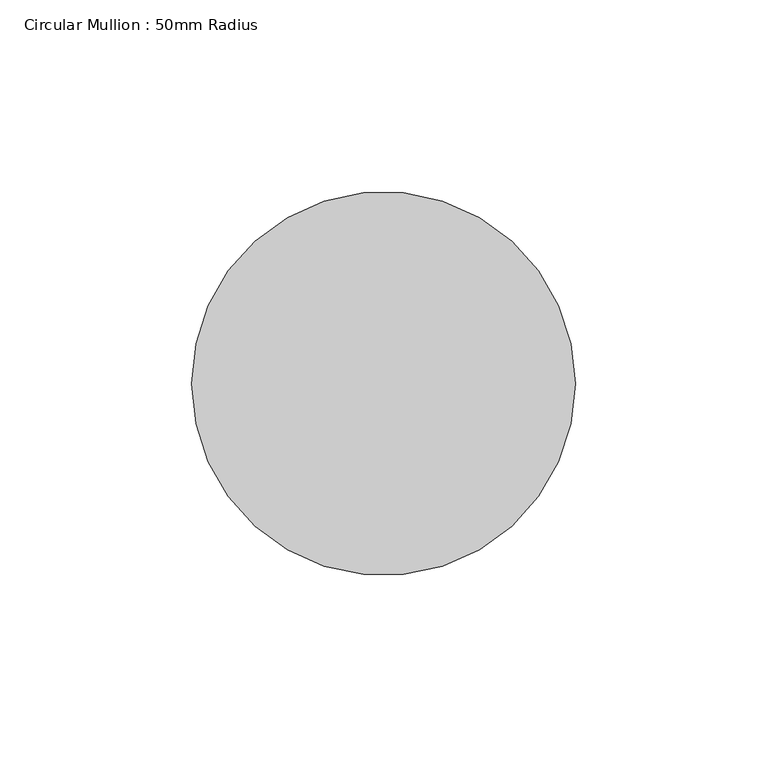
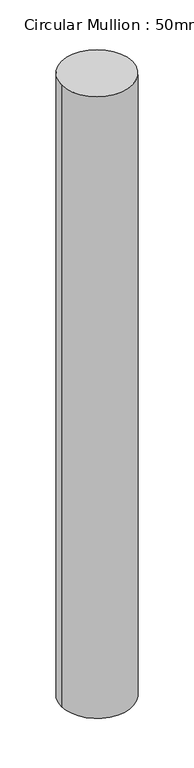
"""IFC4 building model written with IfcOpenShell, lengths in millimetres: member geometry, Circular Mullion : 50mm Radius."""

from ifc_helpers import new_model, si_unit, point, frame, origin, origin_2d, place, context, project, spatial, circle_curve, trimmed, segment, composite_curve, outline, extrude, source, transform, mapped, element, save


def circular_mullion_50mm_radius_4ba9e032(model_context):
    return source(origin(), model_context, "Body", "SweptSolid", [
        extrude(outline(composite_curve([segment(trimmed(circle_curve(origin_2d(), 50.0), [point((50.0, 0.0))], [point((-50.0, 0.0))], False, "CARTESIAN"), True, "CONTINUOUS"), segment(trimmed(circle_curve(origin_2d(), 50.0), [point((-50.0, 0.0))], [point((50.0, 0.0))], False, "CARTESIAN"), True, "CONTINUOUS")], self_intersect=False)), frame((0.0, 0.0, -924.5584625), z_axis=(0.0, 0.0, 1.0), x_axis=(1.0, 0.0, 0.0)), (0.0, 0.0, 1.0), 924.5584625),
    ])


if __name__ == "__main__":
    model = new_model("IFC4")
    model_context = context("Model", 3, world=origin())
    ifc_project = project(units=[si_unit("LENGTHUNIT", "METRE", prefix="MILLI")], contexts=[model_context])
    site = spatial("IfcSite", under=ifc_project)
    building = spatial("IfcBuilding", under=site)
    placement = place(None, origin())
    circular_mullion_50mm_radius_shape = circular_mullion_50mm_radius_4ba9e032(model_context)
    element("IfcMember", 1, ObjectType="Circular Mullion : 50mm Radius", at=placement, inside=building, context=model_context, shape_type="MappedRepresentation", body=[
        mapped(circular_mullion_50mm_radius_shape, transform((0.0, 0.0, 0.0), x_axis=(1.0, 0.0, 0.0), y_axis=(0.0, 1.0, 0.0), z_axis=(0.0, 0.0, 1.0))),
    ])
    save(model, "model.ifc")

# Revit data of these elements
# Type "Circular Mullion : 50mm Radius"
#   built-in parameter 1007350 = 0.164042 (stored number, unit not read)
# Element 1 (IfcMember, "Circular Mullion : 50mm Radius")
#   Materials on its faces: "Aluminium"
# Materials
#   "Aluminium": class "Metal", colour RGB 247 247 247, transparency 0, Description = "Aluminium 6061", Cost = 0
